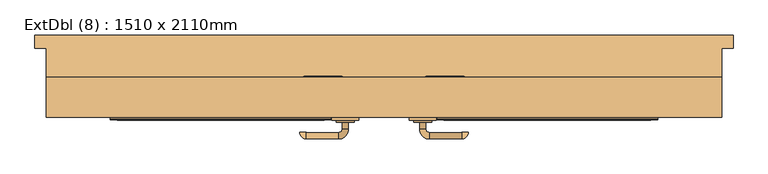
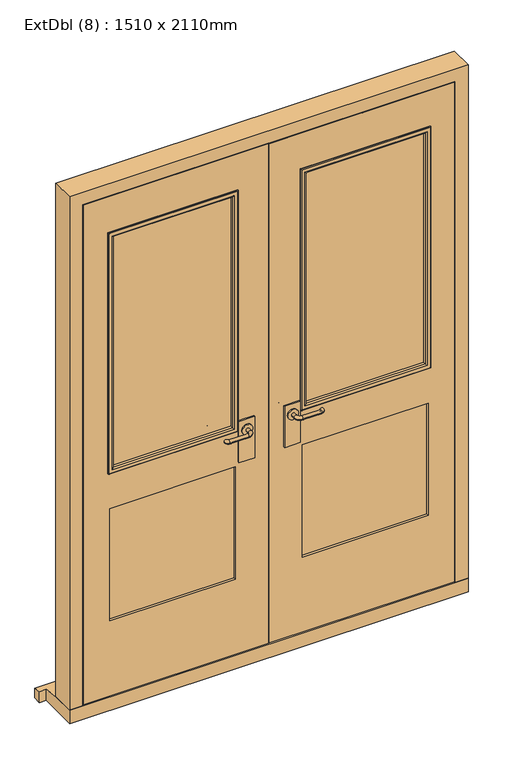
"""IFC4 building model written with IfcOpenShell, lengths in millimetres: door geometry, ExtDbl (8) : 1510 x 2110mm."""

from ifc_helpers import new_model, si_unit, point, frame, frame_2d, origin, place, context, project, spatial, polyline, circle_curve, ellipse_curve, trimmed, segment, composite_curve, outline, extrude, faceted_brep, source, transform, mapped, element, save
from ifc_brep_helpers import plane_surface, cylinder_surface, revolved_surface, advanced_brep


def extdbl_8_1510_x_2110mm_e5df33cb(model_context):
    return source(origin(), model_context, "Body", "SolidModel", [
        extrude(outline(composite_curve([segment(trimmed(circle_curve(frame_2d((950.0, 86.5)), 20.0), [point((950.0, 66.5))], [point((950.0, 106.5))], False, "CARTESIAN"), True, "CONTINUOUS"), segment(trimmed(circle_curve(frame_2d((950.0, 86.5)), 20.0), [point((950.0, 106.5))], [point((950.0, 66.5))], False, "CARTESIAN"), True, "CONTINUOUS")], self_intersect=False)), frame((0.0, 10.4070105, 0.0), z_axis=(0.0, 1.0, 0.0), x_axis=(0.0, 0.0, 1.0)), (0.0, 0.0, 1.0), 4.5929895),
        advanced_brep(
        [(93.5, 10.4070105, 950.0), (79.5, 10.4070105, 950.0), (79.5, -5.0, 950.0), (93.5, -5.0, 950.0), (101.5, -27.0, 950.0), (101.5, -13.0, 950.0), (173.5, -27.0, 950.0), (173.5, -13.0, 950.0), (174.5, -12.0, 950.0), (188.5, -12.0, 950.0)],
        [
            (0, 1, circle_curve(frame((86.5, 10.4070105, 950.0), z_axis=(0.0, 1.0, 0.0), x_axis=(-1.0, 0.0, 0.0)), 7.0)),
            (1, 0, circle_curve(frame((86.5, 10.4070105, 950.0), z_axis=(0.0, 1.0, 0.0), x_axis=(-1.0, 0.0, 0.0)), 7.0)),
            (1, 2),
            (2, 3, circle_curve(frame((86.5, -5.0, 950.0), z_axis=(0.0, 1.0, 0.0), x_axis=(-1.0, 0.0, 0.0)), 7.0)),
            (3, 0),
            (3, 2, circle_curve(frame((86.5, -5.0, 950.0), z_axis=(0.0, 1.0, 0.0), x_axis=(-1.0, 0.0, 0.0)), 7.0)),
            (4, 5, circle_curve(frame((101.5, -20.0, 950.0), z_axis=(-1.0, 0.0, 0.0), x_axis=(0.0, -1.0, 0.0)), 7.0)),
            (5, 3, circle_curve(frame((101.5, -5.0, 950.0), z_axis=(0.0, 0.0, -1.0), x_axis=(-1.0, 0.0, 0.0)), 8.0)),
            (2, 4, circle_curve(frame((101.5, -5.0, 950.0), z_axis=(0.0, 0.0, 1.0), x_axis=(-1.0, 0.0, 0.0)), 22.0)),
            (5, 4, circle_curve(frame((101.5, -20.0, 950.0), z_axis=(-1.0, 0.0, 0.0), x_axis=(0.0, -1.0, 0.0)), 7.0)),
            (4, 6),
            (6, 7, circle_curve(frame((173.5, -20.0, 950.0), z_axis=(-1.0, 0.0, 0.0), x_axis=(0.0, -1.0, 0.0)), 7.0)),
            (7, 5),
            (7, 6, circle_curve(frame((173.5, -20.0, 950.0), z_axis=(-1.0, 0.0, 0.0), x_axis=(0.0, -1.0, 0.0)), 7.0)),
            (8, 9, circle_curve(frame((181.5, -12.0, 950.0), z_axis=(0.0, 1.0, 0.0), x_axis=(1.0, 0.0, 0.0)), 7.0)),
            (9, 8, circle_curve(frame((181.5, -12.0, 950.0), z_axis=(0.0, 1.0, 0.0), x_axis=(1.0, 0.0, 0.0)), 7.0)),
            (8, 7, circle_curve(frame((173.5, -12.0, 950.0), z_axis=(0.0, 0.0, -1.0), x_axis=(0.0, -1.0, 0.0)), 1.0)),
            (6, 9, circle_curve(frame((173.5, -12.0, 950.0), z_axis=(0.0, 0.0, 1.0), x_axis=(0.0, -1.0, 0.0)), 15.0)),
        ],
        [
            plane_surface(frame((86.5, 10.4070105, 950.0), z_axis=(0.0, 1.0, 0.0), x_axis=(0.0, 0.0, 1.0))),
            cylinder_surface(frame((86.5, 10.4070105, 950.0), z_axis=(0.0, 1.0, 0.0), x_axis=(-1.0, 0.0, 0.0)), 7.0),
            revolved_surface(trimmed(ellipse_curve(frame((86.5, -5.0, 950.0), z_axis=(0.0, -1.0, 0.0), x_axis=(-1.0, 0.0, 0.0)), 7.0, 7.0), [point((93.5, -5.0, 950.0))], [point((79.5, -5.0, 950.0))], True, "CARTESIAN"), (101.5, -5.0, 950.0), (0.0, 0.0, -1.0)),
            revolved_surface(trimmed(ellipse_curve(frame((86.5, -5.0, 950.0), z_axis=(0.0, -1.0, 0.0), x_axis=(-1.0, 0.0, 0.0)), 7.0, 7.0), [point((79.5, -5.0, 950.0))], [point((93.5, -5.0, 950.0))], True, "CARTESIAN"), (101.5, -5.0, 950.0), (0.0, 0.0, -1.0)),
            cylinder_surface(frame((101.5, -20.0, 950.0), z_axis=(-1.0, 0.0, 0.0), x_axis=(0.0, -1.0, 0.0)), 7.0),
            plane_surface(frame((181.5, -12.0, 950.0), z_axis=(0.0, 1.0, 0.0), x_axis=(0.0, 0.0, 1.0))),
            revolved_surface(trimmed(ellipse_curve(frame((173.5, -20.0, 950.0), z_axis=(1.0, 0.0, 0.0), x_axis=(0.0, -1.0, 0.0)), 7.0, 7.0), [point((173.5, -13.0, 950.0))], [point((173.5, -27.0, 950.0))], True, "CARTESIAN"), (173.5, -12.0, 950.0), (0.0, 0.0, -1.0)),
            revolved_surface(trimmed(ellipse_curve(frame((173.5, -20.0, 950.0), z_axis=(1.0, 0.0, 0.0), x_axis=(0.0, -1.0, 0.0)), 7.0, 7.0), [point((173.5, -27.0, 950.0))], [point((173.5, -13.0, 950.0))], True, "CARTESIAN"), (173.5, -12.0, 950.0), (0.0, 0.0, -1.0)),
        ],
        [
            (0, [[1, 2]]),
            (1, [[3, 4, 5, -2]]),
            (1, [[-5, 6, -3, -1]]),
            (2, [[7, 8, -4, 9]]),
            (3, [[10, -9, -6, -8]]),
            (4, [[11, 12, 13, -7]]),
            (4, [[-13, 14, -11, -10]]),
            (5, [[15, 16]]),
            (6, [[-15, 17, -12, 18]]),
            (7, [[-16, -18, -14, -17]]),
        ],
    ),
        extrude(outline(polyline([(116.5, 21.0), (116.5, 15.0), (56.5, 15.0), (56.5, 21.0), (116.5, 21.0)])), frame((0.0, 0.0, 825.0), z_axis=(0.0, 0.0, 1.0), x_axis=(1.0, 0.0, 0.0)), (0.0, 0.0, 1.0), 165.0),
        extrude(outline(composite_curve([segment(trimmed(circle_curve(frame_2d((950.0, -86.5)), 20.0), [point((950.0, -66.5))], [point((950.0, -106.5))], False, "CARTESIAN"), True, "CONTINUOUS"), segment(trimmed(circle_curve(frame_2d((950.0, -86.5)), 20.0), [point((950.0, -106.5))], [point((950.0, -66.5))], False, "CARTESIAN"), True, "CONTINUOUS")], self_intersect=False)), frame((0.0, 10.4070105, 0.0), z_axis=(0.0, 1.0, 0.0), x_axis=(0.0, 0.0, 1.0)), (0.0, 0.0, 1.0), 4.5929895),
        advanced_brep(
        [(-93.5, 10.4070105, 950.0), (-79.5, 10.4070105, 950.0), (-93.5, -5.0, 950.0), (-79.5, -5.0, 950.0), (-101.5, -27.0, 950.0), (-101.5, -13.0, 950.0), (-173.5, -13.0, 950.0), (-173.5, -27.0, 950.0), (-174.5, -12.0, 950.0), (-188.5, -12.0, 950.0)],
        [
            (0, 1, circle_curve(frame((-86.5, 10.4070105, 950.0), z_axis=(0.0, 1.0, 0.0), x_axis=(1.0, 0.0, 0.0)), 7.0)),
            (1, 0, circle_curve(frame((-86.5, 10.4070105, 950.0), z_axis=(0.0, 1.0, 0.0), x_axis=(1.0, 0.0, 0.0)), 7.0)),
            (0, 2),
            (2, 3, circle_curve(frame((-86.5, -5.0, 950.0), z_axis=(0.0, 1.0, 0.0), x_axis=(1.0, 0.0, 0.0)), 7.0)),
            (3, 1),
            (3, 2, circle_curve(frame((-86.5, -5.0, 950.0), z_axis=(0.0, 1.0, 0.0), x_axis=(1.0, 0.0, 0.0)), 7.0)),
            (4, 3, circle_curve(frame((-101.5, -5.0, 950.0), z_axis=(0.0, 0.0, 1.0), x_axis=(1.0, 0.0, 0.0)), 22.0)),
            (2, 5, circle_curve(frame((-101.5, -5.0, 950.0), z_axis=(0.0, 0.0, -1.0), x_axis=(1.0, 0.0, 0.0)), 8.0)),
            (5, 4, circle_curve(frame((-101.5, -20.0, 950.0), z_axis=(1.0, 0.0, 0.0), x_axis=(0.0, -1.0, 0.0)), 7.0)),
            (4, 5, circle_curve(frame((-101.5, -20.0, 950.0), z_axis=(1.0, 0.0, 0.0), x_axis=(0.0, -1.0, 0.0)), 7.0)),
            (5, 6),
            (6, 7, circle_curve(frame((-173.5, -20.0, 950.0), z_axis=(1.0, 0.0, 0.0), x_axis=(0.0, -1.0, 0.0)), 7.0)),
            (7, 4),
            (7, 6, circle_curve(frame((-173.5, -20.0, 950.0), z_axis=(1.0, 0.0, 0.0), x_axis=(0.0, -1.0, 0.0)), 7.0)),
            (8, 9, circle_curve(frame((-181.5, -12.0, 950.0), z_axis=(0.0, 1.0, 0.0), x_axis=(-1.0, 0.0, 0.0)), 7.0)),
            (9, 8, circle_curve(frame((-181.5, -12.0, 950.0), z_axis=(0.0, 1.0, 0.0), x_axis=(-1.0, 0.0, 0.0)), 7.0)),
            (9, 7, circle_curve(frame((-173.5, -12.0, 950.0), z_axis=(0.0, 0.0, 1.0), x_axis=(0.0, -1.0, 0.0)), 15.0)),
            (6, 8, circle_curve(frame((-173.5, -12.0, 950.0), z_axis=(0.0, 0.0, -1.0), x_axis=(0.0, -1.0, 0.0)), 1.0)),
        ],
        [
            plane_surface(frame((-86.5, 10.4070105, 950.0), z_axis=(0.0, 1.0, 0.0), x_axis=(0.0, 0.0, 1.0))),
            cylinder_surface(frame((-86.5, 10.4070105, 950.0), z_axis=(0.0, 1.0, 0.0), x_axis=(1.0, 0.0, 0.0)), 7.0),
            revolved_surface(trimmed(ellipse_curve(frame((-86.5, -5.0, 950.0), z_axis=(0.0, 1.0, 0.0), x_axis=(1.0, 0.0, 0.0)), 7.0, 7.0), [point((-93.5, -5.0, 950.0))], [point((-79.5, -5.0, 950.0))], True, "CARTESIAN"), (-101.5, -5.0, 950.0), (0.0, 0.0, -1.0)),
            revolved_surface(trimmed(ellipse_curve(frame((-86.5, -5.0, 950.0), z_axis=(0.0, 1.0, 0.0), x_axis=(1.0, 0.0, 0.0)), 7.0, 7.0), [point((-79.5, -5.0, 950.0))], [point((-93.5, -5.0, 950.0))], True, "CARTESIAN"), (-101.5, -5.0, 950.0), (0.0, 0.0, -1.0)),
            cylinder_surface(frame((-101.5, -20.0, 950.0), z_axis=(1.0, 0.0, 0.0), x_axis=(0.0, -1.0, 0.0)), 7.0),
            plane_surface(frame((-181.5, -12.0, 950.0), z_axis=(0.0, 1.0, 0.0), x_axis=(0.0, 0.0, 1.0))),
            revolved_surface(trimmed(ellipse_curve(frame((-173.5, -20.0, 950.0), z_axis=(1.0, 0.0, 0.0), x_axis=(0.0, -1.0, 0.0)), 7.0, 7.0), [point((-173.5, -13.0, 950.0))], [point((-173.5, -27.0, 950.0))], True, "CARTESIAN"), (-173.5, -12.0, 950.0), (0.0, 0.0, -1.0)),
            revolved_surface(trimmed(ellipse_curve(frame((-173.5, -20.0, 950.0), z_axis=(1.0, 0.0, 0.0), x_axis=(0.0, -1.0, 0.0)), 7.0, 7.0), [point((-173.5, -27.0, 950.0))], [point((-173.5, -13.0, 950.0))], True, "CARTESIAN"), (-173.5, -12.0, 950.0), (0.0, 0.0, -1.0)),
        ],
        [
            (0, [[1, 2]]),
            (1, [[-1, 3, 4, 5]]),
            (1, [[-2, -5, 6, -3]]),
            (2, [[7, -4, 8, 9]]),
            (3, [[-8, -6, -7, 10]]),
            (4, [[-9, 11, 12, 13]]),
            (4, [[-10, -13, 14, -11]]),
            (5, [[15, 16]]),
            (6, [[17, -12, 18, -16]]),
            (7, [[-18, -14, -17, -15]]),
        ],
    ),
        extrude(outline(polyline([(-116.5, 21.0), (-56.5, 21.0), (-56.5, 15.0), (-116.5, 15.0), (-116.5, 21.0)])), frame((0.0, 0.0, 825.0), z_axis=(0.0, 0.0, 1.0), x_axis=(1.0, 0.0, 0.0)), (0.0, 0.0, 1.0), 165.0),
        extrude(outline(composite_curve([segment(trimmed(circle_curve(frame_2d((950.0, -86.5)), 20.0), [point((950.0, -66.5))], [point((950.0, -106.5))], False, "CARTESIAN"), True, "CONTINUOUS"), segment(trimmed(circle_curve(frame_2d((950.0, -86.5)), 20.0), [point((950.0, -106.5))], [point((950.0, -66.5))], False, "CARTESIAN"), True, "CONTINUOUS")], self_intersect=False)), frame((0.0, 71.0, 0.0), z_axis=(0.0, 1.0, 0.0), x_axis=(0.0, 0.0, 1.0)), (0.0, 0.0, 1.0), 4.5929895),
        advanced_brep(
        [(-93.5, 75.5929895, 950.0), (-79.5, 75.5929895, 950.0), (-79.5, 91.0, 950.0), (-93.5, 91.0, 950.0), (-101.5, 113.0, 950.0), (-101.5, 99.0, 950.0), (-173.5, 113.0, 950.0), (-173.5, 99.0, 950.0), (-174.5, 98.0, 950.0), (-188.5, 98.0, 950.0)],
        [
            (0, 1, circle_curve(frame((-86.5, 75.5929895, 950.0), z_axis=(0.0, -1.0, 0.0), x_axis=(1.0, 0.0, 0.0)), 7.0)),
            (1, 0, circle_curve(frame((-86.5, 75.5929895, 950.0), z_axis=(0.0, -1.0, 0.0), x_axis=(1.0, 0.0, 0.0)), 7.0)),
            (1, 2),
            (2, 3, circle_curve(frame((-86.5, 91.0, 950.0), z_axis=(0.0, -1.0, 0.0), x_axis=(1.0, 0.0, 0.0)), 7.0)),
            (3, 0),
            (3, 2, circle_curve(frame((-86.5, 91.0, 950.0), z_axis=(0.0, -1.0, 0.0), x_axis=(1.0, 0.0, 0.0)), 7.0)),
            (4, 5, circle_curve(frame((-101.5, 106.0, 950.0), z_axis=(1.0, 0.0, 0.0), x_axis=(0.0, 1.0, 0.0)), 7.0)),
            (5, 3, circle_curve(frame((-101.5, 91.0, 950.0), z_axis=(0.0, 0.0, -1.0), x_axis=(1.0, 0.0, 0.0)), 8.0)),
            (2, 4, circle_curve(frame((-101.5, 91.0, 950.0), z_axis=(0.0, 0.0, 1.0), x_axis=(1.0, 0.0, 0.0)), 22.0)),
            (5, 4, circle_curve(frame((-101.5, 106.0, 950.0), z_axis=(1.0, 0.0, 0.0), x_axis=(0.0, 1.0, 0.0)), 7.0)),
            (4, 6),
            (6, 7, circle_curve(frame((-173.5, 106.0, 950.0), z_axis=(1.0, 0.0, 0.0), x_axis=(0.0, 1.0, 0.0)), 7.0)),
            (7, 5),
            (7, 6, circle_curve(frame((-173.5, 106.0, 950.0), z_axis=(1.0, 0.0, 0.0), x_axis=(0.0, 1.0, 0.0)), 7.0)),
            (8, 9, circle_curve(frame((-181.5, 98.0, 950.0), z_axis=(0.0, -1.0, 0.0), x_axis=(-1.0, 0.0, 0.0)), 7.0)),
            (9, 8, circle_curve(frame((-181.5, 98.0, 950.0), z_axis=(0.0, -1.0, 0.0), x_axis=(-1.0, 0.0, 0.0)), 7.0)),
            (8, 7, circle_curve(frame((-173.5, 98.0, 950.0), z_axis=(0.0, 0.0, -1.0), x_axis=(0.0, 1.0, 0.0)), 1.0)),
            (6, 9, circle_curve(frame((-173.5, 98.0, 950.0), z_axis=(0.0, 0.0, 1.0), x_axis=(0.0, 1.0, 0.0)), 15.0)),
        ],
        [
            plane_surface(frame((-86.5, 75.5929895, 950.0), z_axis=(0.0, -1.0, 0.0), x_axis=(0.0, 0.0, 1.0))),
            cylinder_surface(frame((-86.5, 75.5929895, 950.0), z_axis=(0.0, -1.0, 0.0), x_axis=(1.0, 0.0, 0.0)), 7.0),
            revolved_surface(trimmed(ellipse_curve(frame((-86.5, 91.0, 950.0), z_axis=(0.0, 1.0, 0.0), x_axis=(1.0, 0.0, 0.0)), 7.0, 7.0), [point((-93.5, 91.0, 950.0))], [point((-79.5, 91.0, 950.0))], True, "CARTESIAN"), (-101.5, 91.0, 950.0), (0.0, 0.0, -1.0)),
            revolved_surface(trimmed(ellipse_curve(frame((-86.5, 91.0, 950.0), z_axis=(0.0, 1.0, 0.0), x_axis=(1.0, 0.0, 0.0)), 7.0, 7.0), [point((-79.5, 91.0, 950.0))], [point((-93.5, 91.0, 950.0))], True, "CARTESIAN"), (-101.5, 91.0, 950.0), (0.0, 0.0, -1.0)),
            cylinder_surface(frame((-101.5, 106.0, 950.0), z_axis=(1.0, 0.0, 0.0), x_axis=(0.0, 1.0, 0.0)), 7.0),
            plane_surface(frame((-181.5, 98.0, 950.0), z_axis=(0.0, -1.0, 0.0), x_axis=(0.0, 0.0, 1.0))),
            revolved_surface(trimmed(ellipse_curve(frame((-173.5, 106.0, 950.0), z_axis=(-1.0, 0.0, 0.0), x_axis=(0.0, 1.0, 0.0)), 7.0, 7.0), [point((-173.5, 99.0, 950.0))], [point((-173.5, 113.0, 950.0))], True, "CARTESIAN"), (-173.5, 98.0, 950.0), (0.0, 0.0, -1.0)),
            revolved_surface(trimmed(ellipse_curve(frame((-173.5, 106.0, 950.0), z_axis=(-1.0, 0.0, 0.0), x_axis=(0.0, 1.0, 0.0)), 7.0, 7.0), [point((-173.5, 113.0, 950.0))], [point((-173.5, 99.0, 950.0))], True, "CARTESIAN"), (-173.5, 98.0, 950.0), (0.0, 0.0, -1.0)),
        ],
        [
            (0, [[1, 2]]),
            (1, [[3, 4, 5, -2]]),
            (1, [[-5, 6, -3, -1]]),
            (2, [[7, 8, -4, 9]]),
            (3, [[10, -9, -6, -8]]),
            (4, [[11, 12, 13, -7]]),
            (4, [[-13, 14, -11, -10]]),
            (5, [[15, 16]]),
            (6, [[-15, 17, -12, 18]]),
            (7, [[-16, -18, -14, -17]]),
        ],
    ),
        extrude(outline(polyline([(-116.5, 65.0), (-116.5, 71.0), (-56.5, 71.0), (-56.5, 65.0), (-116.5, 65.0)])), frame((0.0, 0.0, 825.0), z_axis=(0.0, 0.0, 1.0), x_axis=(1.0, 0.0, 0.0)), (0.0, 0.0, 1.0), 165.0),
        extrude(outline(composite_curve([segment(trimmed(circle_curve(frame_2d((950.0, 86.5)), 20.0), [point((950.0, 66.5))], [point((950.0, 106.5))], False, "CARTESIAN"), True, "CONTINUOUS"), segment(trimmed(circle_curve(frame_2d((950.0, 86.5)), 20.0), [point((950.0, 106.5))], [point((950.0, 66.5))], False, "CARTESIAN"), True, "CONTINUOUS")], self_intersect=False)), frame((0.0, 71.0, 0.0), z_axis=(0.0, 1.0, 0.0), x_axis=(0.0, 0.0, 1.0)), (0.0, 0.0, 1.0), 4.5929895),
        advanced_brep(
        [(93.5, 75.5929895, 950.0), (79.5, 75.5929895, 950.0), (93.5, 91.0, 950.0), (79.5, 91.0, 950.0), (101.5, 113.0, 950.0), (101.5, 99.0, 950.0), (173.5, 99.0, 950.0), (173.5, 113.0, 950.0), (174.5, 98.0, 950.0), (188.5, 98.0, 950.0)],
        [
            (0, 1, circle_curve(frame((86.5, 75.5929895, 950.0), z_axis=(0.0, -1.0, 0.0), x_axis=(-1.0, 0.0, 0.0)), 7.0)),
            (1, 0, circle_curve(frame((86.5, 75.5929895, 950.0), z_axis=(0.0, -1.0, 0.0), x_axis=(-1.0, 0.0, 0.0)), 7.0)),
            (0, 2),
            (2, 3, circle_curve(frame((86.5, 91.0, 950.0), z_axis=(0.0, -1.0, 0.0), x_axis=(-1.0, 0.0, 0.0)), 7.0)),
            (3, 1),
            (3, 2, circle_curve(frame((86.5, 91.0, 950.0), z_axis=(0.0, -1.0, 0.0), x_axis=(-1.0, 0.0, 0.0)), 7.0)),
            (4, 3, circle_curve(frame((101.5, 91.0, 950.0), z_axis=(0.0, 0.0, 1.0), x_axis=(-1.0, 0.0, 0.0)), 22.0)),
            (2, 5, circle_curve(frame((101.5, 91.0, 950.0), z_axis=(0.0, 0.0, -1.0), x_axis=(-1.0, 0.0, 0.0)), 8.0)),
            (5, 4, circle_curve(frame((101.5, 106.0, 950.0), z_axis=(-1.0, 0.0, 0.0), x_axis=(0.0, 1.0, 0.0)), 7.0)),
            (4, 5, circle_curve(frame((101.5, 106.0, 950.0), z_axis=(-1.0, 0.0, 0.0), x_axis=(0.0, 1.0, 0.0)), 7.0)),
            (5, 6),
            (6, 7, circle_curve(frame((173.5, 106.0, 950.0), z_axis=(-1.0, 0.0, 0.0), x_axis=(0.0, 1.0, 0.0)), 7.0)),
            (7, 4),
            (7, 6, circle_curve(frame((173.5, 106.0, 950.0), z_axis=(-1.0, 0.0, 0.0), x_axis=(0.0, 1.0, 0.0)), 7.0)),
            (8, 9, circle_curve(frame((181.5, 98.0, 950.0), z_axis=(0.0, -1.0, 0.0), x_axis=(1.0, 0.0, 0.0)), 7.0)),
            (9, 8, circle_curve(frame((181.5, 98.0, 950.0), z_axis=(0.0, -1.0, 0.0), x_axis=(1.0, 0.0, 0.0)), 7.0)),
            (9, 7, circle_curve(frame((173.5, 98.0, 950.0), z_axis=(0.0, 0.0, 1.0), x_axis=(0.0, 1.0, 0.0)), 15.0)),
            (6, 8, circle_curve(frame((173.5, 98.0, 950.0), z_axis=(0.0, 0.0, -1.0), x_axis=(0.0, 1.0, 0.0)), 1.0)),
        ],
        [
            plane_surface(frame((86.5, 75.5929895, 950.0), z_axis=(0.0, -1.0, 0.0), x_axis=(0.0, 0.0, 1.0))),
            cylinder_surface(frame((86.5, 75.5929895, 950.0), z_axis=(0.0, -1.0, 0.0), x_axis=(-1.0, 0.0, 0.0)), 7.0),
            revolved_surface(trimmed(ellipse_curve(frame((86.5, 91.0, 950.0), z_axis=(0.0, -1.0, 0.0), x_axis=(-1.0, 0.0, 0.0)), 7.0, 7.0), [point((93.5, 91.0, 950.0))], [point((79.5, 91.0, 950.0))], True, "CARTESIAN"), (101.5, 91.0, 950.0), (0.0, 0.0, -1.0)),
            revolved_surface(trimmed(ellipse_curve(frame((86.5, 91.0, 950.0), z_axis=(0.0, -1.0, 0.0), x_axis=(-1.0, 0.0, 0.0)), 7.0, 7.0), [point((79.5, 91.0, 950.0))], [point((93.5, 91.0, 950.0))], True, "CARTESIAN"), (101.5, 91.0, 950.0), (0.0, 0.0, -1.0)),
            cylinder_surface(frame((101.5, 106.0, 950.0), z_axis=(-1.0, 0.0, 0.0), x_axis=(0.0, 1.0, 0.0)), 7.0),
            plane_surface(frame((181.5, 98.0, 950.0), z_axis=(0.0, -1.0, 0.0), x_axis=(0.0, 0.0, 1.0))),
            revolved_surface(trimmed(ellipse_curve(frame((173.5, 106.0, 950.0), z_axis=(-1.0, 0.0, 0.0), x_axis=(0.0, 1.0, 0.0)), 7.0, 7.0), [point((173.5, 99.0, 950.0))], [point((173.5, 113.0, 950.0))], True, "CARTESIAN"), (173.5, 98.0, 950.0), (0.0, 0.0, -1.0)),
            revolved_surface(trimmed(ellipse_curve(frame((173.5, 106.0, 950.0), z_axis=(-1.0, 0.0, 0.0), x_axis=(0.0, 1.0, 0.0)), 7.0, 7.0), [point((173.5, 113.0, 950.0))], [point((173.5, 99.0, 950.0))], True, "CARTESIAN"), (173.5, 98.0, 950.0), (0.0, 0.0, -1.0)),
        ],
        [
            (0, [[1, 2]]),
            (1, [[-1, 3, 4, 5]]),
            (1, [[-2, -5, 6, -3]]),
            (2, [[7, -4, 8, 9]]),
            (3, [[-8, -6, -7, 10]]),
            (4, [[-9, 11, 12, 13]]),
            (4, [[-10, -13, 14, -11]]),
            (5, [[15, 16]]),
            (6, [[17, -12, 18, -16]]),
            (7, [[-18, -14, -17, -15]]),
        ],
    ),
        extrude(outline(polyline([(116.5, 65.0), (56.5, 65.0), (56.5, 71.0), (116.5, 71.0), (116.5, 65.0)])), frame((0.0, 0.0, 825.0), z_axis=(0.0, 0.0, 1.0), x_axis=(1.0, 0.0, 0.0)), (0.0, 0.0, 1.0), 165.0),
        faceted_brep([(684.5, 110.0, 54.5), (755.0, 110.0, 54.5), (755.0, 21.0, 54.5), (706.5, 21.0, 54.5), (706.5, 68.0, 54.5), (684.5, 68.0, 54.5), (684.5, 110.0, 2039.5), (-684.5, 110.0, 2039.5), (-684.5, 110.0, 54.5), (-755.0, 110.0, 54.5), (-755.0, 110.0, 2110.0), (755.0, 110.0, 2110.0), (755.0, 21.0, 2110.0), (-755.0, 21.0, 2110.0), (-755.0, 21.0, 54.5), (-706.5, 21.0, 54.5), (-706.5, 21.0, 2061.5), (706.5, 21.0, 2061.5), (706.5, 68.0, 2061.5), (-706.5, 68.0, 2061.5), (-706.5, 68.0, 54.5), (-684.5, 68.0, 54.5), (-684.5, 68.0, 2039.5), (684.5, 68.0, 2039.5)], [[[0, 1, 2, 3, 4, 5]], [[1, 0, 6, 7, 8, 9, 10, 11]], [[2, 1, 11, 12]], [[3, 2, 12, 13, 14, 15, 16, 17]], [[4, 3, 17, 18]], [[5, 4, 18, 19, 20, 21, 22, 23]], [[0, 5, 23, 6]], [[7, 22, 21, 8]], [[8, 21, 20, 15, 14, 9]], [[13, 10, 9, 14]], [[19, 16, 15, 20]], [[12, 11, 10, 13]], [[18, 17, 16, 19]], [[6, 23, 22, 7]]]),
        extrude(outline(polyline([(603.5, 31.0), (126.5, 31.0), (126.5, 55.0), (603.5, 55.0), (603.5, 31.0)])), frame((0.0, 0.0, 358.5), z_axis=(0.0, 0.0, 1.0), x_axis=(1.0, 0.0, 0.0)), (0.0, 0.0, 1.0), 450.0),
        extrude(outline(polyline([(-126.5, 31.0), (-603.5, 31.0), (-603.5, 55.0), (-126.5, 55.0), (-126.5, 31.0)])), frame((0.0, 0.0, 358.5), z_axis=(0.0, 0.0, 1.0), x_axis=(1.0, 0.0, 0.0)), (0.0, 0.0, 1.0), 450.0),
        extrude(outline(polyline([(126.5, 55.0), (601.9390207, 55.0), (601.9390207, 31.0), (126.5, 31.0), (126.5, 55.0)])), frame((0.0, 0.0, 958.5), z_axis=(0.0, 0.0, 1.0), x_axis=(1.0, 0.0, 0.0)), (0.0, 0.0, 1.0), 950.0),
        extrude(outline(polyline([(-603.5, 55.0), (-126.5, 55.0), (-126.5, 31.0), (-603.5, 31.0), (-603.5, 55.0)])), frame((0.0, 0.0, 958.5), z_axis=(0.0, 0.0, 1.0), x_axis=(1.0, 0.0, 0.0)), (0.0, 0.0, 1.0), 950.0),
        faceted_brep([(780.0, 205.0, 0.0), (780.0, 205.0, 38.5947221), (780.0, 175.0, 43.6174415), (780.0, 175.0, 0.0), (-780.0, 205.0, 38.5947221), (-780.0, 205.0, 0.0), (-780.0, 175.0, 0.0), (-780.0, 175.0, 43.6174415), (755.0, 175.0, 0.0), (755.0, 21.0, 0.0), (-755.0, 21.0, 0.0), (-755.0, 175.0, 0.0), (-755.0, 175.0, 43.6174415), (-755.0, 110.0, 54.5), (755.0, 110.0, 54.5), (755.0, 175.0, 43.6174415), (-755.0, 21.0, 54.5), (755.0, 21.0, 54.5)], [[[0, 1, 2, 3]], [[4, 5, 6, 7]], [[5, 0, 3, 8, 9, 10, 11, 6]], [[1, 0, 5, 4]], [[1, 4, 7, 12, 13, 14, 15, 2]], [[13, 16, 17, 14]], [[16, 10, 9, 17]], [[12, 11, 10, 16, 13]], [[11, 12, 7, 6]], [[8, 15, 14, 17, 9]], [[15, 8, 3, 2]]]),
        extrude(outline(polyline([(58.5, 703.5), (2058.5, 703.5), (2058.5, 1.5), (58.5, 1.5), (58.5, 703.5)]), holes=[polyline([(1908.5, 603.5), (958.5, 603.5), (958.5, 126.5), (1908.5, 126.5), (1908.5, 603.5)]), polyline([(808.5, 126.5), (808.5, 603.5), (358.5, 603.5), (358.5, 126.5), (808.5, 126.5)])]), frame((0.0, 21.0, 0.0), z_axis=(0.0, 1.0, 0.0), x_axis=(0.0, 0.0, 1.0)), (0.0, 0.0, 1.0), 44.0),
        extrude(outline(polyline([(58.5, -703.5), (58.5, -1.5), (2058.5, -1.5), (2058.5, -703.5), (58.5, -703.5)]), holes=[polyline([(1908.5, -126.5), (958.5, -126.5), (958.5, -603.5), (1908.5, -603.5), (1908.5, -126.5)]), polyline([(808.5, -603.5), (808.5, -126.5), (358.5, -126.5), (358.5, -603.5), (808.5, -603.5)])]), frame((0.0, 21.0, 0.0), z_axis=(0.0, 1.0, 0.0), x_axis=(0.0, 0.0, 1.0)), (0.0, 0.0, 1.0), 44.0),
        advanced_brep(
        [(-611.5, 69.0, 950.5), (-611.5, 65.0, 950.5), (-611.5, 65.0, 1916.5), (-611.5, 69.0, 1916.5), (-609.5, 71.0, 952.5), (-609.5, 71.0, 1914.5), (-591.5, 66.0, 970.5), (-596.5, 71.0, 965.5), (-596.5, 71.0, 1901.5), (-591.5, 66.0, 1896.5), (-591.5, 55.0, 970.5), (-591.5, 55.0, 1896.5), (-603.5, 65.0, 958.5), (-603.5, 55.0, 958.5), (-603.5, 55.0, 1908.5), (-603.5, 65.0, 1908.5), (-118.5, 65.0, 1916.5), (-118.5, 69.0, 1916.5), (-120.5, 71.0, 1914.5), (-133.5, 71.0, 1901.5), (-138.5, 66.0, 1896.5), (-138.5, 55.0, 1896.5), (-126.5, 55.0, 1908.5), (-126.5, 65.0, 1908.5), (-118.5, 65.0, 950.5), (-118.5, 69.0, 950.5), (-120.5, 71.0, 952.5), (-133.5, 71.0, 965.5), (-138.5, 66.0, 970.5), (-138.5, 55.0, 970.5), (-126.5, 55.0, 958.5), (-126.5, 65.0, 958.5)],
        [
            (0, 1),
            (1, 2),
            (2, 3),
            (3, 0),
            (4, 0, ellipse_curve(frame((-609.5, 69.0, 952.5), z_axis=(-0.7071067811865472, 0.0, 0.7071067811865477), x_axis=(-0.7071067811865477, 0.0, -0.7071067811865475)), 2.8284271, 2.0)),
            (3, 5, ellipse_curve(frame((-609.5, 69.0, 1914.5), z_axis=(-0.7071067811865475, 0.0, -0.7071067811865475), x_axis=(0.7071067811865474, 0.0, -0.7071067811865476)), 2.8284271, 2.0)),
            (5, 4),
            (6, 7, ellipse_curve(frame((-596.5, 66.0, 965.5), z_axis=(-0.7071067811865472, 0.0, 0.7071067811865477), x_axis=(-0.7071067811865477, 0.0, -0.7071067811865475)), 7.0710678, 5.0)),
            (7, 8),
            (8, 9, ellipse_curve(frame((-596.5, 66.0, 1901.5), z_axis=(-0.7071067811865475, 0.0, -0.7071067811865475), x_axis=(0.7071067811865474, 0.0, -0.7071067811865476)), 7.0710678, 5.0)),
            (9, 6),
            (10, 6),
            (9, 11),
            (11, 10),
            (12, 13),
            (13, 14),
            (14, 15),
            (15, 12),
            (2, 16),
            (16, 17),
            (17, 3),
            (17, 18, ellipse_curve(frame((-120.5, 69.0, 1914.5), z_axis=(-0.7071067811865475, 0.0, 0.7071067811865476), x_axis=(-0.7071067811865476, 0.0, -0.7071067811865475)), 2.8284271, 2.0)),
            (18, 5),
            (8, 19),
            (19, 20, ellipse_curve(frame((-133.5, 66.0, 1901.5), z_axis=(-0.7071067811865475, 0.0, 0.7071067811865476), x_axis=(-0.7071067811865476, 0.0, -0.7071067811865475)), 7.0710678, 5.0)),
            (20, 9),
            (20, 21),
            (21, 11),
            (14, 22),
            (22, 23),
            (23, 15),
            (16, 24),
            (24, 25),
            (25, 17),
            (25, 26, ellipse_curve(frame((-120.5, 69.0, 952.5), z_axis=(0.7071067811865477, 0.0, 0.7071067811865471), x_axis=(-0.707106781186547, 0.0, 0.7071067811865481)), 2.8284271, 2.0)),
            (26, 18),
            (19, 27),
            (27, 28, ellipse_curve(frame((-133.5, 66.0, 965.5), z_axis=(0.7071067811865477, 0.0, 0.7071067811865471), x_axis=(-0.707106781186547, 0.0, 0.7071067811865481)), 7.0710678, 5.0)),
            (28, 20),
            (28, 29),
            (29, 21),
            (22, 30),
            (30, 31),
            (31, 23),
            (24, 1),
            (0, 25),
            (4, 26),
            (7, 27),
            (6, 28),
            (10, 29),
            (13, 30),
            (12, 31),
        ],
        [
            plane_surface(frame((-611.5, 65.0, 950.5), z_axis=(-1.0, 0.0, 0.0), x_axis=(0.0, 0.0, 1.0))),
            cylinder_surface(frame((-609.5, 69.0, 958.5), z_axis=(0.0, 0.0, -1.0), x_axis=(-1.0, 0.0, 0.0)), 2.0),
            cylinder_surface(frame((-596.5, 66.0, 958.5), z_axis=(0.0, 0.0, -1.0), x_axis=(-1.0, 0.0, 0.0)), 5.0),
            plane_surface(frame((-591.5, 66.0, 970.5), z_axis=(1.0, 0.0, 0.0), x_axis=(0.0, 0.0, 1.0))),
            plane_surface(frame((-603.5, 55.0, 958.5), z_axis=(-1.0, 0.0, 0.0), x_axis=(0.0, 0.0, 1.0))),
            plane_surface(frame((-611.5, 65.0, 1916.5), z_axis=(0.0, 0.0, 1.0), x_axis=(1.0, 0.0, 0.0))),
            cylinder_surface(frame((-603.5, 69.0, 1914.5), z_axis=(-1.0, 0.0, 0.0), x_axis=(0.0, 0.0, 1.0)), 2.0),
            cylinder_surface(frame((-603.5, 66.0, 1901.5), z_axis=(-1.0, 0.0, 0.0), x_axis=(0.0, 0.0, 1.0)), 5.0),
            plane_surface(frame((-591.5, 66.0, 1896.5), z_axis=(0.0, 0.0, -1.0), x_axis=(1.0, 0.0, 0.0))),
            plane_surface(frame((-603.5, 55.0, 1908.5), z_axis=(0.0, 0.0, 1.0), x_axis=(1.0, 0.0, 0.0))),
            plane_surface(frame((-118.5, 65.0, 1916.5), z_axis=(1.0, 0.0, 0.0), x_axis=(0.0, 0.0, -1.0))),
            cylinder_surface(frame((-120.5, 69.0, 1908.5), z_axis=(0.0, 0.0, 1.0), x_axis=(1.0, 0.0, 0.0)), 2.0),
            cylinder_surface(frame((-133.5, 66.0, 1908.5), z_axis=(0.0, 0.0, 1.0), x_axis=(1.0, 0.0, 0.0)), 5.0),
            plane_surface(frame((-138.5, 66.0, 1896.5), z_axis=(-1.0, 0.0, 0.0), x_axis=(0.0, 0.0, -1.0))),
            plane_surface(frame((-126.5, 55.0, 1908.5), z_axis=(1.0, 0.0, 0.0), x_axis=(0.0, 0.0, -1.0))),
            plane_surface(frame((-118.5, 65.0, 950.5), z_axis=(0.0, 0.0, -1.0), x_axis=(-1.0, 0.0, 0.0))),
            cylinder_surface(frame((-126.5, 69.0, 952.5), z_axis=(1.0, 0.0, 0.0), x_axis=(0.0, 0.0, -1.0)), 2.0),
            plane_surface(frame((-120.5, 71.0, 952.5), z_axis=(0.0, 1.0, 0.0), x_axis=(-1.0, 0.0, 0.0))),
            cylinder_surface(frame((-126.5, 66.0, 965.5), z_axis=(1.0, 0.0, 0.0), x_axis=(0.0, 0.0, -1.0)), 5.0),
            plane_surface(frame((-138.5, 66.0, 970.5), z_axis=(0.0, 0.0, 1.0), x_axis=(-1.0, 0.0, 0.0))),
            plane_surface(frame((-138.5, 55.0, 970.5), z_axis=(0.0, -1.0, 0.0), x_axis=(-1.0, 0.0, 0.0))),
            plane_surface(frame((-126.5, 55.0, 958.5), z_axis=(0.0, 0.0, -1.0), x_axis=(-1.0, 0.0, 0.0))),
            plane_surface(frame((-126.5, 65.0, 958.5), z_axis=(0.0, -1.0, 0.0), x_axis=(-1.0, 0.0, 0.0))),
        ],
        [
            (0, [[1, 2, 3, 4]]),
            (1, [[5, -4, 6, 7]]),
            (2, [[8, 9, 10, 11]]),
            (3, [[12, -11, 13, 14]]),
            (4, [[15, 16, 17, 18]]),
            (5, [[-3, 19, 20, 21]]),
            (6, [[-6, -21, 22, 23]]),
            (7, [[-10, 24, 25, 26]]),
            (8, [[-13, -26, 27, 28]]),
            (9, [[-17, 29, 30, 31]]),
            (10, [[-20, 32, 33, 34]]),
            (11, [[-22, -34, 35, 36]]),
            (12, [[-25, 37, 38, 39]]),
            (13, [[-27, -39, 40, 41]]),
            (14, [[-30, 42, 43, 44]]),
            (15, [[-33, 45, -1, 46]]),
            (16, [[-35, -46, -5, 47]]),
            (17, [[-23, -36, -47, -7], [48, -37, -24, -9]]),
            (18, [[-38, -48, -8, 49]]),
            (19, [[-40, -49, -12, 50]]),
            (20, [[51, -42, -29, -16], [-28, -41, -50, -14]]),
            (21, [[-43, -51, -15, 52]]),
            (22, [[-45, -32, -19, -2], [-31, -44, -52, -18]]),
        ],
    ),
        advanced_brep(
        [(-126.5, 31.0, 1908.5), (-126.5, 21.0, 1908.5), (-126.5, 21.0, 958.5), (-126.5, 31.0, 958.5), (-138.5, 20.0, 1896.5), (-138.5, 31.0, 1896.5), (-138.5, 31.0, 970.5), (-138.5, 20.0, 970.5), (-133.5, 15.0, 1901.5), (-133.5, 15.0, 965.5), (-118.5, 17.0, 1916.5), (-120.5, 15.0, 1914.5), (-120.5, 15.0, 952.5), (-118.5, 17.0, 950.5), (-118.5, 21.0, 1916.5), (-118.5, 21.0, 950.5), (-603.5, 21.0, 958.5), (-603.5, 31.0, 958.5), (-591.5, 31.0, 970.5), (-591.5, 20.0, 970.5), (-596.5, 15.0, 965.5), (-609.5, 15.0, 952.5), (-611.5, 17.0, 950.5), (-611.5, 21.0, 950.5), (-603.5, 21.0, 1908.5), (-603.5, 31.0, 1908.5), (-591.5, 31.0, 1896.5), (-591.5, 20.0, 1896.5), (-596.5, 15.0, 1901.5), (-609.5, 15.0, 1914.5), (-611.5, 17.0, 1916.5), (-611.5, 21.0, 1916.5)],
        [
            (0, 1),
            (1, 2),
            (2, 3),
            (3, 0),
            (4, 5),
            (5, 6),
            (6, 7),
            (7, 4),
            (8, 4, ellipse_curve(frame((-133.5, 20.0, 1901.5), z_axis=(0.7071067811865475, 0.0, -0.7071067811865475), x_axis=(0.7071067811865474, 0.0, 0.7071067811865476)), 7.0710678, 5.0)),
            (7, 9, ellipse_curve(frame((-133.5, 20.0, 965.5), z_axis=(0.7071067811865475, 0.0, 0.7071067811865475), x_axis=(-0.7071067811865474, 0.0, 0.7071067811865476)), 7.0710678, 5.0)),
            (9, 8),
            (10, 11, ellipse_curve(frame((-120.5, 17.0, 1914.5), z_axis=(0.7071067811865475, 0.0, -0.7071067811865475), x_axis=(0.7071067811865474, 0.0, 0.7071067811865476)), 2.8284271, 2.0)),
            (11, 12),
            (12, 13, ellipse_curve(frame((-120.5, 17.0, 952.5), z_axis=(0.7071067811865475, 0.0, 0.7071067811865475), x_axis=(-0.7071067811865474, 0.0, 0.7071067811865476)), 2.8284271, 2.0)),
            (13, 10),
            (14, 10),
            (13, 15),
            (15, 14),
            (2, 16),
            (16, 17),
            (17, 3),
            (6, 18),
            (18, 19),
            (19, 7),
            (19, 20, ellipse_curve(frame((-596.5, 20.0, 965.5), z_axis=(0.7071067811865475, 0.0, -0.7071067811865475), x_axis=(0.7071067811865476, 0.0, 0.7071067811865474)), 7.0710678, 5.0)),
            (20, 9),
            (12, 21),
            (21, 22, ellipse_curve(frame((-609.5, 17.0, 952.5), z_axis=(0.7071067811865475, 0.0, -0.7071067811865475), x_axis=(0.7071067811865476, 0.0, 0.7071067811865474)), 2.8284271, 2.0)),
            (22, 13),
            (22, 23),
            (23, 15),
            (16, 24),
            (24, 25),
            (25, 17),
            (18, 26),
            (26, 27),
            (27, 19),
            (27, 28, ellipse_curve(frame((-596.5, 20.0, 1901.5), z_axis=(-0.7071067811865475, 0.0, -0.7071067811865475), x_axis=(0.7071067811865474, 0.0, -0.7071067811865476)), 7.0710678, 5.0)),
            (28, 20),
            (21, 29),
            (29, 30, ellipse_curve(frame((-609.5, 17.0, 1914.5), z_axis=(-0.7071067811865475, 0.0, -0.7071067811865475), x_axis=(0.7071067811865474, 0.0, -0.7071067811865476)), 2.8284271, 2.0)),
            (30, 22),
            (30, 31),
            (31, 23),
            (31, 14),
            (1, 24),
            (0, 25),
            (5, 26),
            (4, 27),
            (8, 28),
            (11, 29),
            (10, 30),
        ],
        [
            plane_surface(frame((-126.5, 21.0, 1908.5), z_axis=(1.0, 0.0, 0.0), x_axis=(0.0, 0.0, -1.0))),
            plane_surface(frame((-138.5, 31.0, 1896.5), z_axis=(-1.0, 0.0, 0.0), x_axis=(0.0, 0.0, -1.0))),
            cylinder_surface(frame((-133.5, 20.0, 1908.5), z_axis=(0.0, 0.0, 1.0), x_axis=(1.0, 0.0, 0.0)), 5.0),
            cylinder_surface(frame((-120.5, 17.0, 1908.5), z_axis=(0.0, 0.0, 1.0), x_axis=(1.0, 0.0, 0.0)), 2.0),
            plane_surface(frame((-118.5, 17.0, 1916.5), z_axis=(1.0, 0.0, 0.0), x_axis=(0.0, 0.0, -1.0))),
            plane_surface(frame((-126.5, 21.0, 958.5), z_axis=(0.0, 0.0, -1.0), x_axis=(-1.0, 0.0, 0.0))),
            plane_surface(frame((-138.5, 31.0, 970.5), z_axis=(0.0, 0.0, 1.0), x_axis=(-1.0, 0.0, 0.0))),
            cylinder_surface(frame((-126.5, 20.0, 965.5), z_axis=(1.0, 0.0, 0.0), x_axis=(0.0, 0.0, -1.0)), 5.0),
            cylinder_surface(frame((-126.5, 17.0, 952.5), z_axis=(1.0, 0.0, 0.0), x_axis=(0.0, 0.0, -1.0)), 2.0),
            plane_surface(frame((-118.5, 17.0, 950.5), z_axis=(0.0, 0.0, -1.0), x_axis=(-1.0, 0.0, 0.0))),
            plane_surface(frame((-603.5, 21.0, 958.5), z_axis=(-1.0, 0.0, 0.0), x_axis=(0.0, 0.0, 1.0))),
            plane_surface(frame((-591.5, 31.0, 970.5), z_axis=(1.0, 0.0, 0.0), x_axis=(0.0, 0.0, 1.0))),
            cylinder_surface(frame((-596.5, 20.0, 958.5), z_axis=(0.0, 0.0, -1.0), x_axis=(-1.0, 0.0, 0.0)), 5.0),
            cylinder_surface(frame((-609.5, 17.0, 958.5), z_axis=(0.0, 0.0, -1.0), x_axis=(-1.0, 0.0, 0.0)), 2.0),
            plane_surface(frame((-611.5, 17.0, 950.5), z_axis=(-1.0, 0.0, 0.0), x_axis=(0.0, 0.0, 1.0))),
            plane_surface(frame((-611.5, 21.0, 1916.5), z_axis=(0.0, 1.0, 0.0), x_axis=(1.0, 0.0, 0.0))),
            plane_surface(frame((-603.5, 21.0, 1908.5), z_axis=(0.0, 0.0, 1.0), x_axis=(1.0, 0.0, 0.0))),
            plane_surface(frame((-603.5, 31.0, 1908.5), z_axis=(0.0, 1.0, 0.0), x_axis=(1.0, 0.0, 0.0))),
            plane_surface(frame((-591.5, 31.0, 1896.5), z_axis=(0.0, 0.0, -1.0), x_axis=(1.0, 0.0, 0.0))),
            cylinder_surface(frame((-603.5, 20.0, 1901.5), z_axis=(-1.0, 0.0, 0.0), x_axis=(0.0, 0.0, 1.0)), 5.0),
            plane_surface(frame((-596.5, 15.0, 1901.5), z_axis=(0.0, -1.0, 0.0), x_axis=(1.0, 0.0, 0.0))),
            cylinder_surface(frame((-603.5, 17.0, 1914.5), z_axis=(-1.0, 0.0, 0.0), x_axis=(0.0, 0.0, 1.0)), 2.0),
            plane_surface(frame((-611.5, 17.0, 1916.5), z_axis=(0.0, 0.0, 1.0), x_axis=(1.0, 0.0, 0.0))),
        ],
        [
            (0, [[1, 2, 3, 4]]),
            (1, [[5, 6, 7, 8]]),
            (2, [[9, -8, 10, 11]]),
            (3, [[12, 13, 14, 15]]),
            (4, [[16, -15, 17, 18]]),
            (5, [[-3, 19, 20, 21]]),
            (6, [[-7, 22, 23, 24]]),
            (7, [[-10, -24, 25, 26]]),
            (8, [[-14, 27, 28, 29]]),
            (9, [[-17, -29, 30, 31]]),
            (10, [[-20, 32, 33, 34]]),
            (11, [[-23, 35, 36, 37]]),
            (12, [[-25, -37, 38, 39]]),
            (13, [[-28, 40, 41, 42]]),
            (14, [[-30, -42, 43, 44]]),
            (15, [[-31, -44, 45, -18], [46, -32, -19, -2]]),
            (16, [[-33, -46, -1, 47]]),
            (17, [[-21, -34, -47, -4], [48, -35, -22, -6]]),
            (18, [[-36, -48, -5, 49]]),
            (19, [[-38, -49, -9, 50]]),
            (20, [[51, -40, -27, -13], [-26, -39, -50, -11]]),
            (21, [[-41, -51, -12, 52]]),
            (22, [[-43, -52, -16, -45]]),
        ],
    ),
        advanced_brep(
        [(603.5, 31.0, 1908.5), (603.5, 21.0, 1908.5), (603.5, 21.0, 958.5), (603.5, 31.0, 958.5), (591.5, 20.0, 1896.5), (591.5, 31.0, 1896.5), (591.5, 31.0, 970.5), (591.5, 20.0, 970.5), (596.5, 15.0, 1901.5), (596.5, 15.0, 965.5), (611.5, 17.0, 1916.5), (609.5, 15.0, 1914.5), (609.5, 15.0, 952.5), (611.5, 17.0, 950.5), (611.5, 21.0, 1916.5), (611.5, 21.0, 950.5), (126.5, 21.0, 958.5), (126.5, 31.0, 958.5), (138.5, 31.0, 970.5), (138.5, 20.0, 970.5), (133.5, 15.0, 965.5), (120.5, 15.0, 952.5), (118.5, 17.0, 950.5), (118.5, 21.0, 950.5), (126.5, 21.0, 1908.5), (126.5, 31.0, 1908.5), (138.5, 31.0, 1896.5), (138.5, 20.0, 1896.5), (133.5, 15.0, 1901.5), (120.5, 15.0, 1914.5), (118.5, 17.0, 1916.5), (118.5, 21.0, 1916.5)],
        [
            (0, 1),
            (1, 2),
            (2, 3),
            (3, 0),
            (4, 5),
            (5, 6),
            (6, 7),
            (7, 4),
            (8, 4, ellipse_curve(frame((596.5, 20.0, 1901.5), z_axis=(0.7071067811865519, 0.0, -0.707106781186543), x_axis=(0.707106781186543, 0.0, 0.7071067811865521)), 7.0710678, 5.0)),
            (7, 9, ellipse_curve(frame((596.5, 20.0, 965.5), z_axis=(0.707106781186543, 0.0, 0.707106781186552), x_axis=(-0.707106781186552, 0.0, 0.707106781186543)), 7.0710678, 5.0)),
            (9, 8),
            (10, 11, ellipse_curve(frame((609.5, 17.0, 1914.5), z_axis=(0.7071067811865519, 0.0, -0.707106781186543), x_axis=(0.707106781186543, 0.0, 0.7071067811865521)), 2.8284271, 2.0)),
            (11, 12),
            (12, 13, ellipse_curve(frame((609.5, 17.0, 952.5), z_axis=(0.707106781186543, 0.0, 0.707106781186552), x_axis=(-0.707106781186552, 0.0, 0.707106781186543)), 2.8284271, 2.0)),
            (13, 10),
            (14, 10),
            (13, 15),
            (15, 14),
            (2, 16),
            (16, 17),
            (17, 3),
            (6, 18),
            (18, 19),
            (19, 7),
            (19, 20, ellipse_curve(frame((133.5, 20.0, 965.5), z_axis=(0.7071067811865519, 0.0, -0.707106781186543), x_axis=(0.7071067811865432, 0.0, 0.7071067811865517)), 7.0710678, 5.0)),
            (20, 9),
            (12, 21),
            (21, 22, ellipse_curve(frame((120.5, 17.0, 952.5), z_axis=(0.7071067811865519, 0.0, -0.707106781186543), x_axis=(0.7071067811865432, 0.0, 0.7071067811865517)), 2.8284271, 2.0)),
            (22, 13),
            (22, 23),
            (23, 15),
            (16, 24),
            (24, 25),
            (25, 17),
            (18, 26),
            (26, 27),
            (27, 19),
            (27, 28, ellipse_curve(frame((133.5, 20.0, 1901.5), z_axis=(-0.7071067811865431, 0.0, -0.7071067811865518), x_axis=(0.7071067811865517, 0.0, -0.7071067811865432)), 7.0710678, 5.0)),
            (28, 20),
            (21, 29),
            (29, 30, ellipse_curve(frame((120.5, 17.0, 1914.5), z_axis=(-0.7071067811865431, 0.0, -0.7071067811865518), x_axis=(0.7071067811865517, 0.0, -0.7071067811865432)), 2.8284271, 2.0)),
            (30, 22),
            (30, 31),
            (31, 23),
            (31, 14),
            (1, 24),
            (0, 25),
            (5, 26),
            (4, 27),
            (8, 28),
            (11, 29),
            (10, 30),
        ],
        [
            plane_surface(frame((603.5, 21.0, 1908.5), z_axis=(1.0, 0.0, 0.0), x_axis=(0.0, 0.0, -1.0))),
            plane_surface(frame((591.5, 31.0, 1896.5), z_axis=(-1.0, 0.0, 0.0), x_axis=(0.0, 0.0, -1.0))),
            cylinder_surface(frame((596.5, 20.0, 1908.5), z_axis=(0.0, 0.0, 1.0), x_axis=(1.0, 0.0, 0.0)), 5.0),
            cylinder_surface(frame((609.5, 17.0, 1908.5), z_axis=(0.0, 0.0, 1.0), x_axis=(1.0, 0.0, 0.0)), 2.0),
            plane_surface(frame((611.5, 17.0, 1916.5), z_axis=(1.0, 0.0, 0.0), x_axis=(0.0, 0.0, -1.0))),
            plane_surface(frame((603.5, 21.0, 958.5), z_axis=(0.0, 0.0, -1.0), x_axis=(-1.0, 0.0, 0.0))),
            plane_surface(frame((591.5, 31.0, 970.5), z_axis=(0.0, 0.0, 1.0), x_axis=(-1.0, 0.0, 0.0))),
            cylinder_surface(frame((603.5, 20.0, 965.5), z_axis=(1.0, 0.0, 0.0), x_axis=(0.0, 0.0, -1.0)), 5.0),
            cylinder_surface(frame((603.5, 17.0, 952.5), z_axis=(1.0, 0.0, 0.0), x_axis=(0.0, 0.0, -1.0)), 2.0),
            plane_surface(frame((611.5, 17.0, 950.5), z_axis=(0.0, 0.0, -1.0), x_axis=(-1.0, 0.0, 0.0))),
            plane_surface(frame((126.5, 21.0, 958.5), z_axis=(-1.0, 0.0, 0.0), x_axis=(0.0, 0.0, 1.0))),
            plane_surface(frame((138.5, 31.0, 970.5), z_axis=(1.0, 0.0, 0.0), x_axis=(0.0, 0.0, 1.0))),
            cylinder_surface(frame((133.5, 20.0, 958.5), z_axis=(0.0, 0.0, -1.0), x_axis=(-1.0, 0.0, 0.0)), 5.0),
            cylinder_surface(frame((120.5, 17.0, 958.5), z_axis=(0.0, 0.0, -1.0), x_axis=(-1.0, 0.0, 0.0)), 2.0),
            plane_surface(frame((118.5, 17.0, 950.5), z_axis=(-1.0, 0.0, 0.0), x_axis=(0.0, 0.0, 1.0))),
            plane_surface(frame((118.5, 21.0, 1916.5), z_axis=(0.0, 1.0, 0.0), x_axis=(1.0, 0.0, 0.0))),
            plane_surface(frame((126.5, 21.0, 1908.5), z_axis=(0.0, 0.0, 1.0), x_axis=(1.0, 0.0, 0.0))),
            plane_surface(frame((126.5, 31.0, 1908.5), z_axis=(0.0, 1.0, 0.0), x_axis=(1.0, 0.0, 0.0))),
            plane_surface(frame((138.5, 31.0, 1896.5), z_axis=(0.0, 0.0, -1.0), x_axis=(1.0, 0.0, 0.0))),
            cylinder_surface(frame((126.5, 20.0, 1901.5), z_axis=(-1.0, 0.0, 0.0), x_axis=(0.0, 0.0, 1.0)), 5.0),
            plane_surface(frame((133.5, 15.0, 1901.5), z_axis=(0.0, -1.0, 0.0), x_axis=(1.0, 0.0, 0.0))),
            cylinder_surface(frame((126.5, 17.0, 1914.5), z_axis=(-1.0, 0.0, 0.0), x_axis=(0.0, 0.0, 1.0)), 2.0),
            plane_surface(frame((118.5, 17.0, 1916.5), z_axis=(0.0, 0.0, 1.0), x_axis=(1.0, 0.0, 0.0))),
        ],
        [
            (0, [[1, 2, 3, 4]]),
            (1, [[5, 6, 7, 8]]),
            (2, [[9, -8, 10, 11]]),
            (3, [[12, 13, 14, 15]]),
            (4, [[16, -15, 17, 18]]),
            (5, [[-3, 19, 20, 21]]),
            (6, [[-7, 22, 23, 24]]),
            (7, [[-10, -24, 25, 26]]),
            (8, [[-14, 27, 28, 29]]),
            (9, [[-17, -29, 30, 31]]),
            (10, [[-20, 32, 33, 34]]),
            (11, [[-23, 35, 36, 37]]),
            (12, [[-25, -37, 38, 39]]),
            (13, [[-28, 40, 41, 42]]),
            (14, [[-30, -42, 43, 44]]),
            (15, [[-31, -44, 45, -18], [46, -32, -19, -2]]),
            (16, [[-33, -46, -1, 47]]),
            (17, [[-21, -34, -47, -4], [48, -35, -22, -6]]),
            (18, [[-36, -48, -5, 49]]),
            (19, [[-38, -49, -9, 50]]),
            (20, [[51, -40, -27, -13], [-26, -39, -50, -11]]),
            (21, [[-41, -51, -12, 52]]),
            (22, [[-43, -52, -16, -45]]),
        ],
    ),
        advanced_brep(
        [(118.5, 69.0, 950.5), (118.5, 65.0, 950.5), (118.5, 65.0, 1916.5), (118.5, 69.0, 1916.5), (120.5, 71.0, 952.5), (120.5, 71.0, 1914.5), (138.5, 66.0, 970.5), (133.5, 71.0, 965.5), (133.5, 71.0, 1901.5), (138.5, 66.0, 1896.5), (138.5, 55.0, 970.5), (138.5, 55.0, 1896.5), (126.5, 65.0, 958.5), (126.5, 55.0, 958.5), (126.5, 55.0, 1908.5), (126.5, 65.0, 1908.5), (611.5, 65.0, 1916.5), (611.5, 69.0, 1916.5), (609.5, 71.0, 1914.5), (596.5, 71.0, 1901.5), (591.5, 66.0, 1896.5), (591.5, 55.0, 1896.5), (603.5, 55.0, 1908.5), (603.5, 65.0, 1908.5), (611.5, 65.0, 950.5), (611.5, 69.0, 950.5), (609.5, 71.0, 952.5), (596.5, 71.0, 965.5), (591.5, 66.0, 970.5), (591.5, 55.0, 970.5), (603.5, 55.0, 958.5), (603.5, 65.0, 958.5)],
        [
            (0, 1),
            (1, 2),
            (2, 3),
            (3, 0),
            (4, 0, ellipse_curve(frame((120.5, 69.0, 952.5), z_axis=(-0.7071067811865474, 0.0, 0.7071067811865476), x_axis=(-0.7071067811865475, 0.0, -0.7071067811865475)), 2.8284271, 2.0)),
            (3, 5, ellipse_curve(frame((120.5, 69.0, 1914.5), z_axis=(-0.7071067811865476, 0.0, -0.7071067811865474), x_axis=(0.7071067811865471, 0.0, -0.7071067811865478)), 2.8284271, 2.0)),
            (5, 4),
            (6, 7, ellipse_curve(frame((133.5, 66.0, 965.5), z_axis=(-0.7071067811865474, 0.0, 0.7071067811865476), x_axis=(-0.7071067811865475, 0.0, -0.7071067811865475)), 7.0710678, 5.0)),
            (7, 8),
            (8, 9, ellipse_curve(frame((133.5, 66.0, 1901.5), z_axis=(-0.7071067811865476, 0.0, -0.7071067811865474), x_axis=(0.7071067811865471, 0.0, -0.7071067811865478)), 7.0710678, 5.0)),
            (9, 6),
            (10, 6),
            (9, 11),
            (11, 10),
            (12, 13),
            (13, 14),
            (14, 15),
            (15, 12),
            (2, 16),
            (16, 17),
            (17, 3),
            (17, 18, ellipse_curve(frame((609.5, 69.0, 1914.5), z_axis=(-0.7071067811865474, 0.0, 0.7071067811865476), x_axis=(-0.7071067811865478, 0.0, -0.7071067811865472)), 2.8284271, 2.0)),
            (18, 5),
            (8, 19),
            (19, 20, ellipse_curve(frame((596.5, 66.0, 1901.5), z_axis=(-0.7071067811865474, 0.0, 0.7071067811865476), x_axis=(-0.7071067811865478, 0.0, -0.7071067811865472)), 7.0710678, 5.0)),
            (20, 9),
            (20, 21),
            (21, 11),
            (14, 22),
            (22, 23),
            (23, 15),
            (16, 24),
            (24, 25),
            (25, 17),
            (25, 26, ellipse_curve(frame((609.5, 69.0, 952.5), z_axis=(0.7071067811865476, 0.0, 0.7071067811865474), x_axis=(-0.7071067811865472, 0.0, 0.7071067811865478)), 2.8284271, 2.0)),
            (26, 18),
            (19, 27),
            (27, 28, ellipse_curve(frame((596.5, 66.0, 965.5), z_axis=(0.7071067811865476, 0.0, 0.7071067811865474), x_axis=(-0.7071067811865472, 0.0, 0.7071067811865478)), 7.0710678, 5.0)),
            (28, 20),
            (28, 29),
            (29, 21),
            (22, 30),
            (30, 31),
            (31, 23),
            (24, 1),
            (0, 25),
            (4, 26),
            (7, 27),
            (6, 28),
            (10, 29),
            (13, 30),
            (12, 31),
        ],
        [
            plane_surface(frame((118.5, 65.0, 950.5), z_axis=(-1.0, 0.0, 0.0), x_axis=(0.0, 0.0, 1.0))),
            cylinder_surface(frame((120.5, 69.0, 958.5), z_axis=(0.0, 0.0, -1.0), x_axis=(-1.0, 0.0, 0.0)), 2.0),
            cylinder_surface(frame((133.5, 66.0, 958.5), z_axis=(0.0, 0.0, -1.0), x_axis=(-1.0, 0.0, 0.0)), 5.0),
            plane_surface(frame((138.5, 66.0, 970.5), z_axis=(1.0, 0.0, 0.0), x_axis=(0.0, 0.0, 1.0))),
            plane_surface(frame((126.5, 55.0, 958.5), z_axis=(-1.0, 0.0, 0.0), x_axis=(0.0, 0.0, 1.0))),
            plane_surface(frame((118.5, 65.0, 1916.5), z_axis=(0.0, 0.0, 1.0), x_axis=(1.0, 0.0, 0.0))),
            cylinder_surface(frame((126.5, 69.0, 1914.5), z_axis=(-1.0, 0.0, 0.0), x_axis=(0.0, 0.0, 1.0)), 2.0),
            cylinder_surface(frame((126.5, 66.0, 1901.5), z_axis=(-1.0, 0.0, 0.0), x_axis=(0.0, 0.0, 1.0)), 5.0),
            plane_surface(frame((138.5, 66.0, 1896.5), z_axis=(0.0, 0.0, -1.0), x_axis=(1.0, 0.0, 0.0))),
            plane_surface(frame((126.5, 55.0, 1908.5), z_axis=(0.0, 0.0, 1.0), x_axis=(1.0, 0.0, 0.0))),
            plane_surface(frame((611.5, 65.0, 1916.5), z_axis=(1.0, 0.0, 0.0), x_axis=(0.0, 0.0, -1.0))),
            cylinder_surface(frame((609.5, 69.0, 1908.5), z_axis=(0.0, 0.0, 1.0), x_axis=(1.0, 0.0, 0.0)), 2.0),
            cylinder_surface(frame((596.5, 66.0, 1908.5), z_axis=(0.0, 0.0, 1.0), x_axis=(1.0, 0.0, 0.0)), 5.0),
            plane_surface(frame((591.5, 66.0, 1896.5), z_axis=(-1.0, 0.0, 0.0), x_axis=(0.0, 0.0, -1.0))),
            plane_surface(frame((603.5, 55.0, 1908.5), z_axis=(1.0, 0.0, 0.0), x_axis=(0.0, 0.0, -1.0))),
            plane_surface(frame((611.5, 65.0, 950.5), z_axis=(0.0, 0.0, -1.0), x_axis=(-1.0, 0.0, 0.0))),
            cylinder_surface(frame((603.5, 69.0, 952.5), z_axis=(1.0, 0.0, 0.0), x_axis=(0.0, 0.0, -1.0)), 2.0),
            plane_surface(frame((609.5, 71.0, 952.5), z_axis=(0.0, 1.0, 0.0), x_axis=(-1.0, 0.0, 0.0))),
            cylinder_surface(frame((603.5, 66.0, 965.5), z_axis=(1.0, 0.0, 0.0), x_axis=(0.0, 0.0, -1.0)), 5.0),
            plane_surface(frame((591.5, 66.0, 970.5), z_axis=(0.0, 0.0, 1.0), x_axis=(-1.0, 0.0, 0.0))),
            plane_surface(frame((591.5, 55.0, 970.5), z_axis=(0.0, -1.0, 0.0), x_axis=(-1.0, 0.0, 0.0))),
            plane_surface(frame((603.5, 55.0, 958.5), z_axis=(0.0, 0.0, -1.0), x_axis=(-1.0, 0.0, 0.0))),
            plane_surface(frame((603.5, 65.0, 958.5), z_axis=(0.0, -1.0, 0.0), x_axis=(-1.0, 0.0, 0.0))),
        ],
        [
            (0, [[1, 2, 3, 4]]),
            (1, [[5, -4, 6, 7]]),
            (2, [[8, 9, 10, 11]]),
            (3, [[12, -11, 13, 14]]),
            (4, [[15, 16, 17, 18]]),
            (5, [[-3, 19, 20, 21]]),
            (6, [[-6, -21, 22, 23]]),
            (7, [[-10, 24, 25, 26]]),
            (8, [[-13, -26, 27, 28]]),
            (9, [[-17, 29, 30, 31]]),
            (10, [[-20, 32, 33, 34]]),
            (11, [[-22, -34, 35, 36]]),
            (12, [[-25, 37, 38, 39]]),
            (13, [[-27, -39, 40, 41]]),
            (14, [[-30, 42, 43, 44]]),
            (15, [[-33, 45, -1, 46]]),
            (16, [[-35, -46, -5, 47]]),
            (17, [[-23, -36, -47, -7], [48, -37, -24, -9]]),
            (18, [[-38, -48, -8, 49]]),
            (19, [[-40, -49, -12, 50]]),
            (20, [[51, -42, -29, -16], [-28, -41, -50, -14]]),
            (21, [[-43, -51, -15, 52]]),
            (22, [[-45, -32, -19, -2], [-31, -44, -52, -18]]),
        ],
    ),
    ])


if __name__ == "__main__":
    model = new_model("IFC4")
    model_context = context("Model", 3, world=origin())
    ifc_project = project(units=[si_unit("LENGTHUNIT", "METRE", prefix="MILLI")], contexts=[model_context])
    site = spatial("IfcSite", under=ifc_project)
    building = spatial("IfcBuilding", under=site)
    placement = place(None, origin())
    extdbl_8_1510_x_2110mm_shape = extdbl_8_1510_x_2110mm_e5df33cb(model_context)
    element("IfcDoor", 1, ObjectType="ExtDbl (8) : 1510 x 2110mm", at=placement, inside=building, context=model_context, shape_type="MappedRepresentation", body=[
        mapped(extdbl_8_1510_x_2110mm_shape, transform((0.0, 0.0, 0.0), x_axis=(1.0, 0.0, 0.0), y_axis=(0.0, 1.0, 0.0), z_axis=(0.0, 0.0, 1.0))),
    ])
    save(model, "model.ifc")

# Revit data of these elements
# Type "ExtDbl (8) : 1510 x 2110mm"
#   Type Mark = "13"
#   Type Comments = "External Double"
#   Operation = "DoubleDoorSingleSwing"
#   Keynote = "L20"
#   Wrap Layers (Int) from Ext = 177.5 mm
#   Wrap Layers (Ext) from Ext = 102.5 mm
#   Top of Lock Rail = 900 mm
#   Thickness = 44 mm
#   Stile Shutting = 125 mm
#   Stile - Top Rail = 150 mm
#   Stile - Lock Rail = 150 mm
#   Stile - Hanging = 100 mm
#   Stile - Bottom Rail = 300 mm
#   Rough Width = 1510 mm
#   Rough Height = 2110 mm
#   O/A Frame Width = 64 mm
#   Handle Z Distance = 950 mm
#   Glazing Thickness = 24 mm
#   FrameWidth = 42 mm
#   FrameOffset - External = 65 mm
#   FrameDepth = 89 mm
#   Door Panel Width = 702 mm
#   Door Panel Thickness = 44 mm
#   Door Panel Height = 2000 mm
#   Cill Thickness = 54.5 mm
#   Cill Projection = 30 mm
#   Handle X Distance = 75 mm
#   Height = 2110 mm
#   Structural Tolerance = 6.5 mm
#   Tolerance = 3 mm
#   Undercut = 4 mm
#   Width = 1510 mm
#   Cill Extension = 25 mm
#   Cavity Closer Width = 50 mm
#   Cavity Closer Offset from Ext = 102.5 mm
#   Cavity Closer Depth = 85 mm
#   Vis - Ironmongery = yes
#   Vis - Cavity Closers = yes
#   Function = 1
#   Material Glass = Door - Glazing
#   Handle Style = element 171650
#   Material Door = Door - Panel
#   Material Frame = Door - Frame/Mullion
#   Material Ironmongery = Door - Handle
#   Wall Closure = (empty or 0)
# Element 1 (IfcDoor, "ExtDbl (8) : 1510 x 2110mm")
#   Materials on its faces: "Door - Panel", "Door - Handle", "Door - Frame/Mullion", "Door - Glazing"
# Materials
#   "Door - Glazing": class "Miscellaneous", colour RGB 0 0 255, transparency 0.75
#   "Door - Panel": class "Wood", colour RGB 210 159 95, transparency 0
#   "Door - Frame/Mullion": class "Wood", colour RGB 212 179 113, transparency 0
#   "Door - Handle": class "Miscellaneous", colour RGB 247 247 247, transparency 0
